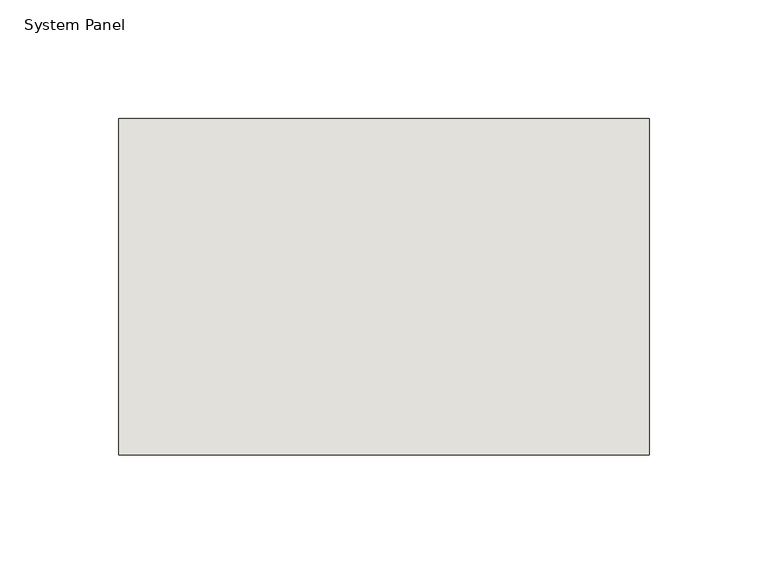
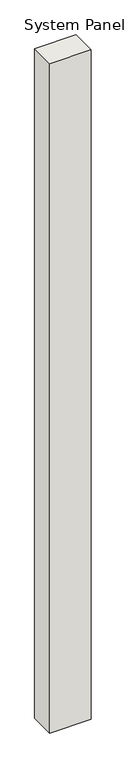
"""IFC4 building model written with IfcOpenShell, lengths in millimetres: wall geometry, System Panel : NLRS_21_CWP_hsb-vulling minerale wol 142 _gen_rsf."""

from ifc_helpers import new_model, si_unit, origin, origin_with_axes, place, context, project, spatial, polyline, outline, extrude, source, transform, mapped, element, save


def system_panel_59c625bf(model_context):
    return source(origin(), model_context, "Body", "SweptSolid", [
        extrude(outline(polyline([(111.9999998, -71.0), (-111.9999998, -71.0), (-111.9999998, 71.0), (111.9999998, 71.0), (111.9999998, -71.0)])), origin_with_axes(), (0.0, 0.0, 1.0), 3849.0),
    ])


if __name__ == "__main__":
    model = new_model("IFC4")
    model_context = context("Model", 3, world=origin())
    ifc_project = project(units=[si_unit("LENGTHUNIT", "METRE", prefix="MILLI")], contexts=[model_context])
    site = spatial("IfcSite", under=ifc_project)
    building = spatial("IfcBuilding", under=site)
    placement = place(None, origin())
    system_panel_shape = system_panel_59c625bf(model_context)
    element("IfcWall", 1, ObjectType="System Panel : NLRS_21_CWP_hsb-vulling minerale wol 142 _gen_rsf", at=placement, inside=building, context=model_context, shape_type="MappedRepresentation", body=[
        mapped(system_panel_shape, transform((0.0, 0.0, 0.0), x_axis=(1.0, 0.0, 0.0), y_axis=(0.0, 1.0, 0.0), z_axis=(0.0, 0.0, 1.0))),
    ])
    save(model, "model.ifc")

# Revit data of these elements
# Type "System Panel : NLRS_21_CWP_hsb-vulling minerale wol 142 _gen_rsf"
#   Type IfcGUID = "07M7mRoiH1CR8m_RSKIwpC"
#   Assembly Code = "21.23"
#   IfcExportAs = "IfcWall"
# Element 1 (IfcWall, "System Panel : NLRS_21_CWP_hsb-vulling minerale wol 142 _gen_rsf")
#   Materials on its faces: "NLRS_m1_isolatie minerale wol_gen_rsf"
# Materials
#   "NLRS_m1_isolatie minerale wol_gen_rsf": class "M - Anorganische materialen", colour RGB 200 200 140, transparency 0, Keynote = "m1", Manufacturer = "Revit Standards Foundation", URL = "www.revitstandards.org", Description = "isolatie minerale wol", Cost = 0
